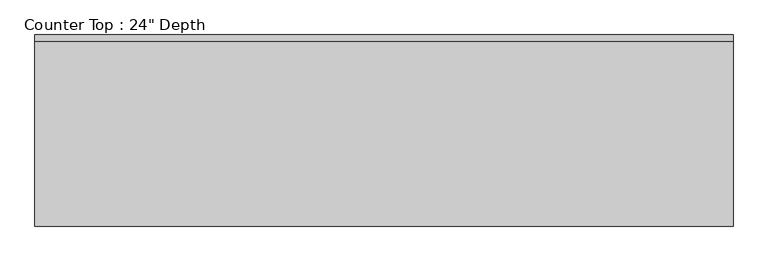
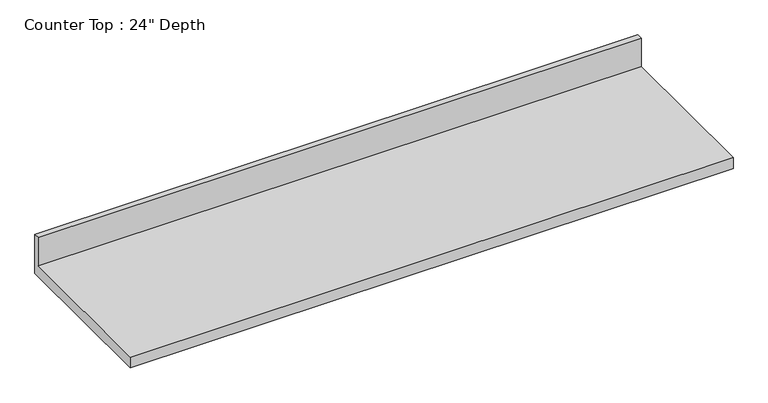
"""IFC4 building model written with IfcOpenShell, lengths in millimetres: furniture geometry."""

import ifcopenshell
import ifcopenshell.guid

model = None  # the IFC model being written
_history = None  # IfcOwnerHistory: only IFC2X3 demands one
_inside = {}  # id of a spatial element -> (the spatial element, [elements in it])
_under = {}  # id of a project, library or spatial element -> (it, [spatial elements below it])
_declared = {}  # id of a project -> (the project, [libraries it declares])
_typed = {}  # id of a type object -> (the type object, [elements of that type])
_made_of = {}  # id of a material, layer set ... -> (it, [elements and type objects made of it])


def new_model(schema):
    """Start an empty IFC model of exactly this schema.

    Asked for "IFC4X3", IfcOpenShell would pick the latest addendum, in which some entities
    have other attributes; the version numbers below select the first issue.
    IFC2X3 requires an IfcOwnerHistory on every rooted entity: one is made here for all.
    """
    global model, _history
    if schema == "IFC4X3":
        model = ifcopenshell.file(schema_version=(4, 3, 0, 0))
    else:
        model = ifcopenshell.file(schema=schema)
    _inside.clear()
    _under.clear()
    _declared.clear()
    _typed.clear()
    _made_of.clear()
    _history = None
    if model.schema == "IFC2X3":
        org = make("IfcOrganization", Name="unknown")
        user = make(
            "IfcPersonAndOrganization",
            ThePerson=make("IfcPerson", FamilyName="unknown"),
            TheOrganization=org,
        )
        app = make(
            "IfcApplication",
            ApplicationDeveloper=org,
            Version="unknown",
            ApplicationFullName="unknown",
            ApplicationIdentifier="unknown",
        )
        _history = make(
            "IfcOwnerHistory",
            OwningUser=user,
            OwningApplication=app,
            ChangeAction="ADDED",
            CreationDate=0,
        )
    return model


def make(cls, **values):
    """One entity of the class cls with the attributes given. An attribute that is None is left unset."""
    return model.create_entity(
        cls, **{name: value for name, value in values.items() if value is not None}
    )


def rooted(cls, **values):
    """An entity with a GlobalId (a new one), such as an element, a storey or a relation."""
    return make(cls, GlobalId=ifcopenshell.guid.new(), OwnerHistory=_history, **values)


def si_unit(unit_type, name, prefix=None):
    """IfcSIUnit, for example si_unit("LENGTHUNIT", "METRE", prefix="MILLI")."""
    return make("IfcSIUnit", UnitType=unit_type, Prefix=prefix, Name=name)


def assignment(units):
    """IfcUnitAssignment: the units of a project."""
    return None if units is None else make("IfcUnitAssignment", Units=units)


def point(xyz):
    """IfcCartesianPoint."""
    return None if xyz is None else make("IfcCartesianPoint", Coordinates=xyz)


def direction(xyz):
    """IfcDirection."""
    return None if xyz is None else make("IfcDirection", DirectionRatios=xyz)


def frame(location, z_axis=None, x_axis=None):
    """IfcAxis2Placement3D, a coordinate frame: its origin and axes. An axis left out is left unset."""
    return make(
        "IfcAxis2Placement3D",
        Location=point(location),
        Axis=direction(z_axis),
        RefDirection=direction(x_axis),
    )


def origin():
    """The frame at (0, 0, 0) with its axes left unset."""
    return frame((0.0, 0.0, 0.0))


def place(relative_to, where):
    """IfcLocalPlacement: puts the frame where relative to a parent placement (None: the world)."""
    return make(
        "IfcLocalPlacement", PlacementRelTo=relative_to, RelativePlacement=where
    )


def context(
    kind, dimensions, precision=None, world=None, true_north=None, identifier=None
):
    """IfcGeometricRepresentationContext, for example the 3D "Model" context."""
    return make(
        "IfcGeometricRepresentationContext",
        ContextIdentifier=identifier,
        ContextType=kind,
        CoordinateSpaceDimension=dimensions,
        Precision=precision,
        WorldCoordinateSystem=world,
        TrueNorth=true_north,
    )


def project(units=None, contexts=None):
    """IfcProject with its units and contexts."""
    return rooted(
        "IfcProject",
        Name="project",
        RepresentationContexts=contexts,
        UnitsInContext=assignment(units),
    )


def spatial(cls, under=None, at=None, **own):
    """A site, building, storey or space (cls), placed at a placement, below another one or the project."""
    s = rooted(cls, ObjectPlacement=at, **own)
    if under is not None:
        _under.setdefault(under.id(), (under, []))[1].append(s)
    return s


def polyline(points):
    """IfcPolyline through the points."""
    return make("IfcPolyline", Points=[point(p) for p in points])


def outline(outer, holes=None, kind="AREA"):
    """IfcArbitraryClosedProfileDef: a profile drawn as a closed curve; with holes, ...WithVoids."""
    if holes is None:
        return make("IfcArbitraryClosedProfileDef", ProfileType=kind, OuterCurve=outer)
    return make(
        "IfcArbitraryProfileDefWithVoids",
        ProfileType=kind,
        OuterCurve=outer,
        InnerCurves=holes,
    )


def extrude(swept, where, along, depth):
    """IfcExtrudedAreaSolid: the profile swept, set in the frame where, extruded along a direction by depth."""
    return make(
        "IfcExtrudedAreaSolid",
        SweptArea=swept,
        Position=where,
        ExtrudedDirection=direction(along),
        Depth=depth,
    )


def shape(context_of_items, identifier, shape_type, items):
    """IfcShapeRepresentation: the items that make up one representation, for example the "Body"."""
    return make(
        "IfcShapeRepresentation",
        ContextOfItems=context_of_items,
        RepresentationIdentifier=identifier,
        RepresentationType=shape_type,
        Items=items,
    )


def source(mapping_origin, context_of_items, identifier, shape_type, items):
    """IfcRepresentationMap: a shape defined once, which mapped items show again and again."""
    return make(
        "IfcRepresentationMap",
        MappingOrigin=mapping_origin,
        MappedRepresentation=shape(context_of_items, identifier, shape_type, items),
    )


def transform(
    local_origin,
    x_axis=None,
    y_axis=None,
    z_axis=None,
    scale=None,
    scale2=None,
    scale3=None,
    uniform=True,
):
    """IfcCartesianTransformationOperator3D, or its non-uniform kind. x_axis, y_axis, z_axis: its Axis1, 2, 3."""
    if uniform:
        return make(
            "IfcCartesianTransformationOperator3D",
            Axis1=direction(x_axis),
            Axis2=direction(y_axis),
            LocalOrigin=point(local_origin),
            Scale=scale,
            Axis3=direction(z_axis),
        )
    return make(
        "IfcCartesianTransformationOperator3DnonUniform",
        Axis1=direction(x_axis),
        Axis2=direction(y_axis),
        LocalOrigin=point(local_origin),
        Scale=scale,
        Axis3=direction(z_axis),
        Scale2=scale2,
        Scale3=scale3,
    )


def mapped(mapping_source, mapping_target):
    """IfcMappedItem: shows the shape of a source again, moved by a transform."""
    return make(
        "IfcMappedItem", MappingSource=mapping_source, MappingTarget=mapping_target
    )


def made_of(thing, what):
    """Note that an element or type object is made of a material, layer set ...; save() writes the relation."""
    if what is not None:
        _made_of.setdefault(what.id(), (what, []))[1].append(thing)
    return thing


def element(
    cls,
    number,
    at=None,
    inside=None,
    cuts=None,
    type_object=None,
    material=None,
    context=None,
    identifier="Body",
    shape_type=None,
    held_by="IfcProductDefinitionShape",
    body=None,
    shapes=None,
    **own,
):
    """One element of the class cls, such as IfcWall. Its Tag is "e" and its number.

    at: its placement. inside: the storey or other place that contains it. cuts: it is an
    opening in that element (IfcRelVoidsElement). A single representation is given by context,
    identifier, shape_type and body (its items); several are given by shapes. held_by: the class
    of the entity that holds the representations. save() writes the other relations.
    """
    e = rooted(cls, Tag="e%d" % number, ObjectPlacement=at, **own)
    if body is not None:
        shapes = [shape(context, identifier, shape_type, body)]
    if shapes is not None:
        e.Representation = make(held_by, Representations=shapes)
    if inside is not None:
        _inside.setdefault(inside.id(), (inside, []))[1].append(e)
    if cuts is not None:
        rooted(
            "IfcRelVoidsElement", RelatingBuildingElement=cuts, RelatedOpeningElement=e
        )
    if type_object is not None:
        _typed.setdefault(type_object.id(), (type_object, []))[1].append(e)
    return made_of(e, material)


def aggregate(whole, parts):
    """IfcRelAggregates: a whole, such as a stair, and the parts it consists of."""
    return rooted("IfcRelAggregates", RelatingObject=whole, RelatedObjects=parts)


def save(model, path):
    """Write the relations noted so far, then the file.

    IfcRelAggregates (storeys below a building ...), IfcRelContainedInSpatialStructure (elements
    in a storey), IfcRelDefinesByType, IfcRelAssociatesMaterial and IfcRelDeclares: one each for
    every whole, place, type object, material and project.
    """
    for whole, parts in _under.values():
        aggregate(whole, parts)
    for where, things in _inside.values():
        rooted(
            "IfcRelContainedInSpatialStructure",
            RelatedElements=things,
            RelatingStructure=where,
        )
    for kind, things in _typed.values():
        rooted("IfcRelDefinesByType", RelatedObjects=things, RelatingType=kind)
    for what, things in _made_of.values():
        rooted("IfcRelAssociatesMaterial", RelatedObjects=things, RelatingMaterial=what)
    for by, libraries in _declared.values():
        rooted("IfcRelDeclares", RelatingContext=by, RelatedDefinitions=libraries)
    model.write(path)


def furniture_ef5f263e(model_context):
    return source(origin(), model_context, "Body", "SweptSolid", [
        extrude(outline(polyline([(0.0, 1016.0), (0.0, 876.3), (-558.8, 876.3), (-558.8, 914.4), (-19.05, 914.4), (-19.05, 1016.0), (0.0, 1016.0)])), frame((-1200.4622951, 0.0, 0.0), z_axis=(1.0, 0.0, 0.0), x_axis=(0.0, 1.0, 0.0)), (0.0, 0.0, 1.0), 2041.525),
    ])


if __name__ == "__main__":
    model = new_model("IFC4")
    model_context = context("Model", 3, world=origin())
    ifc_project = project(units=[si_unit("LENGTHUNIT", "METRE", prefix="MILLI")], contexts=[model_context])
    site = spatial("IfcSite", under=ifc_project)
    building = spatial("IfcBuilding", under=site)
    placement = place(None, origin())
    furniture_shape = furniture_ef5f263e(model_context)
    element("IfcFurniture", 1, ObjectType="Counter Top : 24\" Depth", at=placement, inside=building, context=model_context, shape_type="MappedRepresentation", body=[
        mapped(furniture_shape, transform((0.0, 0.0, 0.0), x_axis=(1.0, 0.0, 0.0), y_axis=(0.0, 1.0, 0.0), z_axis=(0.0, 0.0, 1.0))),
    ])
    save(model, "model.ifc")

# Revit data of these elements
# Type "Counter Top : 24\" Depth"
#   Keynote = "M12366116.01"
#   Assembly Code = "C1030400"
#   Counter Thickness = 0' - 1 1/2"
#   Depth = 1' - 10"
#   Height = 3' - 0"
#   Length [instance default] = 8' - 0"
#   Counter Top Material = none
# Element 1 (IfcFurniture, "Counter Top : 24\" Depth")
#   Length = 6' - 8 3/8"
